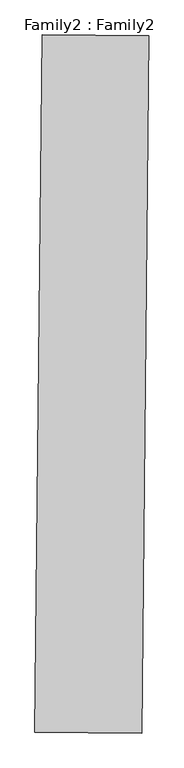
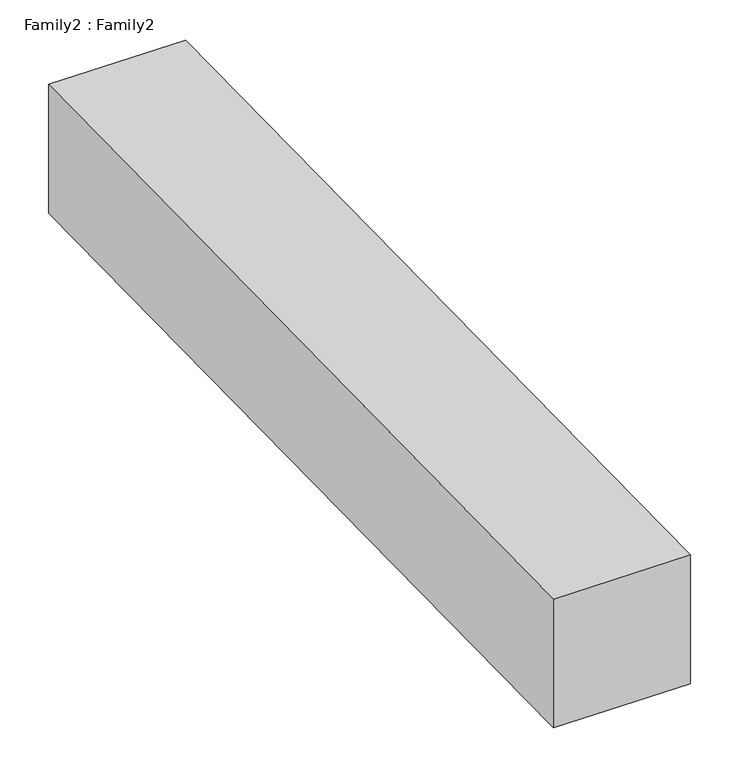
"""IFC4 building model written with IfcOpenShell, lengths in millimetres: proxy geometry, Family2 : Family2."""

from ifc_helpers import new_model, si_unit, origin, place, context, project, spatial, faceted_brep, source, transform, mapped, element, save


def family2_family2_2e7ed927(model_context):
    return source(origin(), model_context, "Body", "Brep", [
        faceted_brep([(-3950.3725143, -6727.5645197, 1.0945136), (-3950.3725143, -6727.5645197, 201.0945136), (-3936.4702802, -5420.0356029, 202.060409), (-3936.4702802, -5420.0356029, 2.060409), (-3750.3813243, -6729.4417323, 201.0945136), (-3736.4790902, -5421.9128156, 202.060409), (-3750.3813243, -6729.4417323, 1.0945136), (-3736.4790902, -5421.9128156, 2.060409)], [[[0, 1, 2, 3]], [[1, 4, 5, 2]], [[4, 6, 7, 5]], [[6, 0, 3, 7]], [[3, 2, 5, 7]], [[0, 6, 4, 1]]]),
    ])


if __name__ == "__main__":
    model = new_model("IFC4")
    model_context = context("Model", 3, world=origin())
    ifc_project = project(units=[si_unit("LENGTHUNIT", "METRE", prefix="MILLI")], contexts=[model_context])
    site = spatial("IfcSite", under=ifc_project)
    building = spatial("IfcBuilding", under=site)
    placement = place(None, origin())
    family2_family2_shape = family2_family2_2e7ed927(model_context)
    element("IfcBuildingElementProxy", 1, Name="Family2 : Family2", ObjectType="Family2 : Family2", at=placement, inside=building, context=model_context, shape_type="MappedRepresentation", body=[
        mapped(family2_family2_shape, transform((0.0, 0.0, 0.0), x_axis=(1.0, 0.0, 0.0), y_axis=(0.0, 1.0, 0.0), z_axis=(0.0, 0.0, 1.0))),
    ])
    save(model, "model.ifc")

# Revit data of these elements
# Type "Family2 : Family2"
#   Default Elevation = 0
